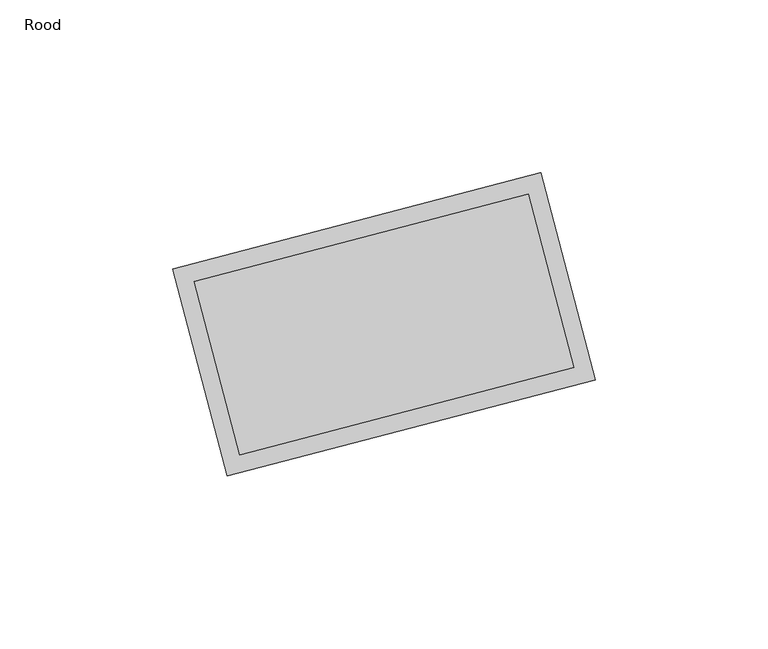
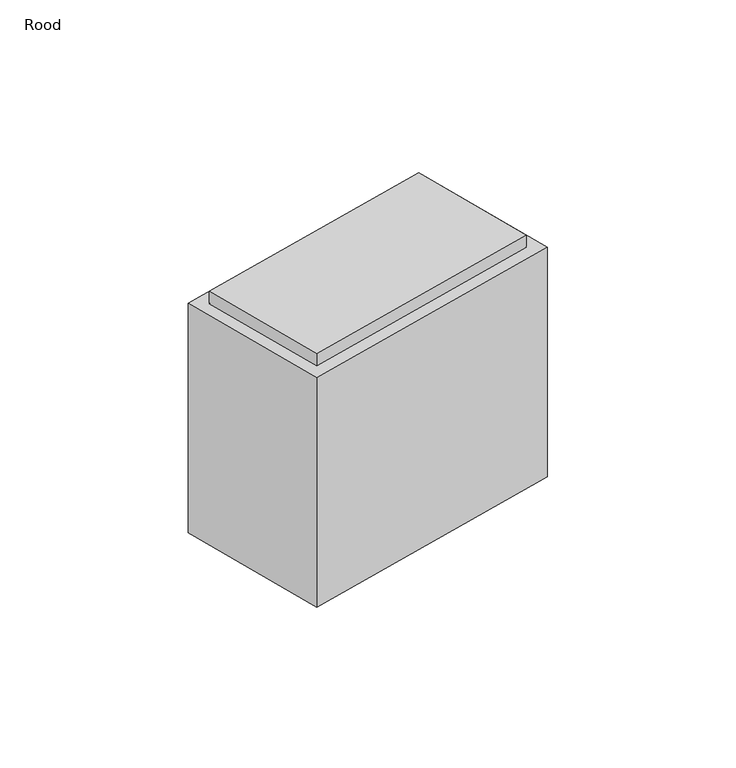
"""IFC4 building model written with IfcOpenShell, lengths in millimetres: proxy geometry, 00_GMA_steen_versie_6 : Rood."""

from ifc_helpers import new_model, si_unit, origin, origin_with_axes, place, context, project, spatial, polyline, outline, extrude, source, transform, mapped, element, save


def rood_14a66368(model_context):
    return source(origin(), model_context, "Body", "SweptSolid", [
        extrude(outline(polyline([(24.8461542, 24.0369432), (9.1731432, 83.919349), (115.5141152, 111.7519519), (131.1871262, 51.8695461), (24.8461542, 24.0369432)]), holes=[polyline([(125.0840527, 55.4406095), (111.9430518, 105.6488784), (15.2762167, 80.3482856), (28.4172176, 30.1400167), (125.0840527, 55.4406095)])]), origin_with_axes(), (0.0, 0.0, 1.0), 95.0),
        extrude(outline(polyline([(111.9430518, 105.6488784), (125.0840527, 55.4406095), (28.4172176, 30.1400167), (15.2762167, 80.3482856), (111.9430518, 105.6488784)])), origin_with_axes(), (0.0, 0.0, 1.0), 100.0),
    ])


if __name__ == "__main__":
    model = new_model("IFC4")
    model_context = context("Model", 3, world=origin())
    ifc_project = project(units=[si_unit("LENGTHUNIT", "METRE", prefix="MILLI")], contexts=[model_context])
    site = spatial("IfcSite", under=ifc_project)
    building = spatial("IfcBuilding", under=site)
    placement = place(None, origin())
    rood_shape = rood_14a66368(model_context)
    element("IfcBuildingElementProxy", 1, Name="00_GMA_steen_versie_6 : Rood", ObjectType="00_GMA_steen_versie_6 : Rood", at=placement, inside=building, context=model_context, shape_type="MappedRepresentation", body=[
        mapped(rood_shape, transform((0.0, 0.0, 0.0), x_axis=(1.0, 0.0, 0.0), y_axis=(0.0, 1.0, 0.0), z_axis=(0.0, 0.0, 1.0))),
    ])
    save(model, "model.ifc")

# Revit data of these elements
# Type "00_GMA_steen_versie_6 : Rood"
#   Voegdikte = 95 mm
#   VoegTovSteen = -5 mm
#   StootvoegLinksHalfOnder [instance default] = 5 mm
#   StootvoegLinksHalfBoven [instance default] = 5 mm
#   StootVoegRechtsHalfOnder [instance default] = 5 mm
#   StootVoegRechtsHalfBoven [instance default] = 5 mm
#   StootVoegBreedteRechts [instance default] = 10 mm
#   StootVoegBreedteLinks [instance default] = 10 mm
#   Steendikte = 100 mm
#   LintVoegOnderHalf [instance default] = 0 mm
#   LintVoegOnder [instance default] = 0 mm
#   LintVoegBovenHalf [instance default] = 5 mm
#   LintVoegBoven [instance default] = 10 mm
#   materiaal = 21_steen_rood
#   MateriaalVoeg = 20_voeg
#   Default Elevation = 0
# Element 1 (IfcBuildingElementProxy, "00_GMA_steen_versie_6 : Rood")
#   LintVoegOnderHalf = 5 mm
#   LintVoegOnder = 10 mm
#   Materials on its faces: "20_voeg", "21_steen_rood"
# Materials
#   "21_steen_rood": class "Unassigned", colour RGB 213 111 43, transparency 0, Cost = 0
#   "20_voeg": class "Concrete", colour RGB 86 86 86, transparency 0, Manufacturer = "RevitGG", URL = "www.revitgg.nl", Description = "zandcement, generiek materiaal", Cost = 0
